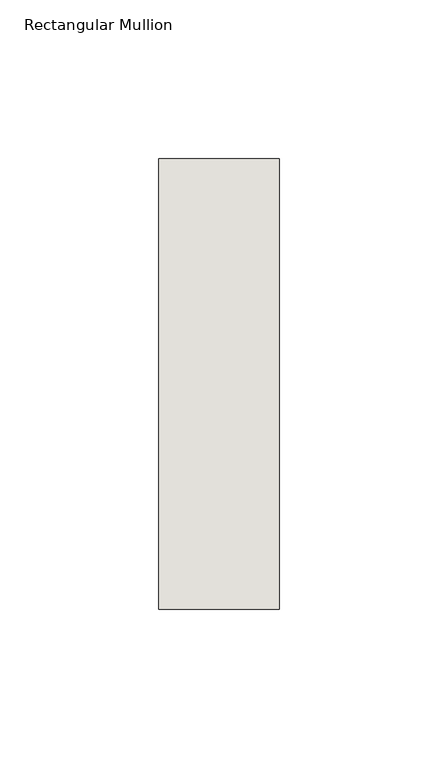
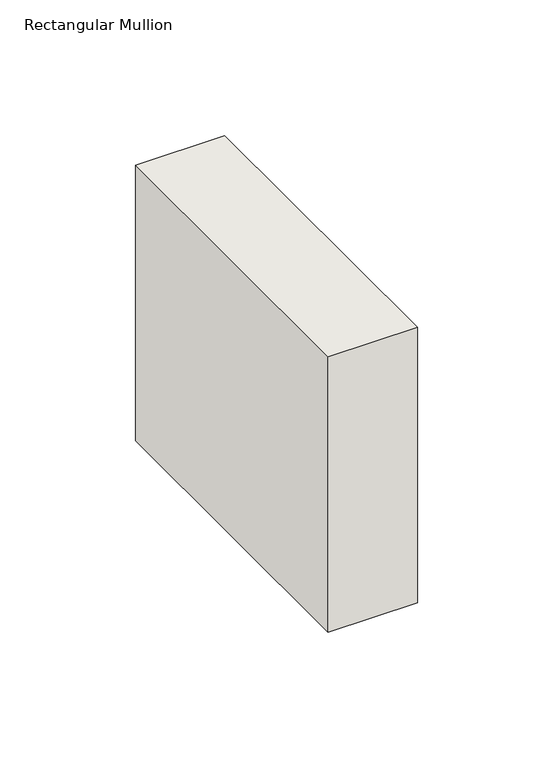
"""IFC4 building model written with IfcOpenShell, lengths in millimetres: wall geometry, Rectangular Mullion : NLRS_21_CWM_hsb-regel 38x142_gen_rsf."""

from ifc_helpers import new_model, si_unit, frame, origin, place, context, project, spatial, polyline, outline, extrude, source, transform, mapped, element, save


def rectangular_mullion_21a1eeaa(model_context):
    return source(origin(), model_context, "Body", "SweptSolid", [
        extrude(outline(polyline([(-38.0, -71.0), (-38.0, 71.0), (0.0, 71.0), (0.0, -71.0), (-38.0, -71.0)])), frame((0.0, 0.0, -123.9999997), z_axis=(0.0, 0.0, 1.0), x_axis=(1.0, 0.0, 0.0)), (0.0, 0.0, 1.0), 123.9999997),
    ])


if __name__ == "__main__":
    model = new_model("IFC4")
    model_context = context("Model", 3, world=origin())
    ifc_project = project(units=[si_unit("LENGTHUNIT", "METRE", prefix="MILLI")], contexts=[model_context])
    site = spatial("IfcSite", under=ifc_project)
    building = spatial("IfcBuilding", under=site)
    placement = place(None, origin())
    rectangular_mullion_shape = rectangular_mullion_21a1eeaa(model_context)
    element("IfcWall", 1, ObjectType="Rectangular Mullion : NLRS_21_CWM_hsb-regel 38x142_gen_rsf", at=placement, inside=building, context=model_context, shape_type="MappedRepresentation", body=[
        mapped(rectangular_mullion_shape, transform((0.0, 0.0, 0.0), x_axis=(1.0, 0.0, 0.0), y_axis=(0.0, 1.0, 0.0), z_axis=(0.0, 0.0, 1.0))),
    ])
    save(model, "model.ifc")

# Revit data of these elements
# Type "Rectangular Mullion : NLRS_21_CWM_hsb-regel 38x142_gen_rsf"
#   Type IfcGUID = "07M7mRoiH1CR8m_RSKIwpF"
#   Assembly Code = "21.10"
#   IfcExportAs = "IfcWall"
#   built-in parameter 1007322 = 0.465879 (stored number, unit not read)
#   built-in parameter 1007321 = 0.062336 (stored number, unit not read)
#   built-in parameter 1007320 = 0.062336 (stored number, unit not read)
# Element 1 (IfcWall, "Rectangular Mullion : NLRS_21_CWM_hsb-regel 38x142_gen_rsf")
#   Materials on its faces: "NLRS_i2_hout naaldhout vuren_gen_rsf"
# Materials
#   "NLRS_i2_hout naaldhout vuren_gen_rsf": class "I - Hout", colour RGB 234 199 147, transparency 0, Keynote = "i2", Manufacturer = "Revit Standards Foundation", URL = "www.revitstandards.org", Description = "hout vuren", Cost = 0
